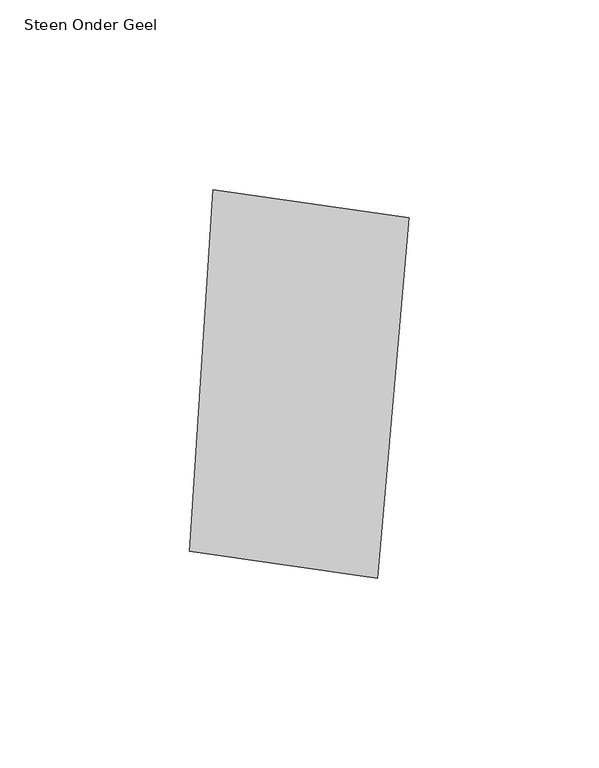
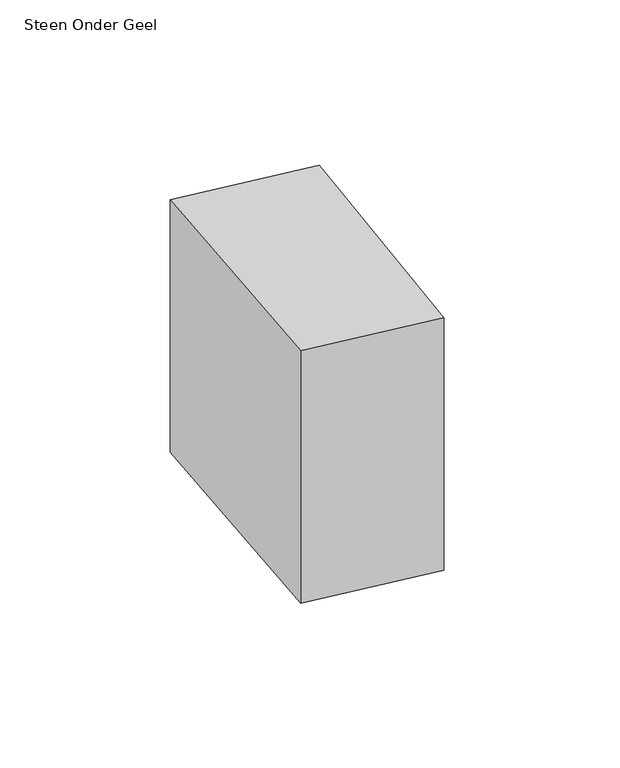
"""IFC4 building model written with IfcOpenShell, lengths in millimetres: proxy geometry, 00_GMA_steen_versie_4 : Steen Onder Geel."""

from ifc_helpers import new_model, si_unit, origin, origin_with_axes, place, context, project, spatial, polyline, outline, extrude, source, transform, mapped, element, save


def steen_onder_geel_60102d9a(model_context):
    return source(origin(), model_context, "Body", "SweptSolid", [
        extrude(outline(polyline([(104.4913091, 114.212909), (96.2842343, 19.4127052), (46.7864635, 26.4817004), (52.9037693, 121.5865884), (104.4913091, 114.212909)])), origin_with_axes(), (0.0, 0.0, 1.0), 100.0),
    ])


if __name__ == "__main__":
    model = new_model("IFC4")
    model_context = context("Model", 3, world=origin())
    ifc_project = project(units=[si_unit("LENGTHUNIT", "METRE", prefix="MILLI")], contexts=[model_context])
    site = spatial("IfcSite", under=ifc_project)
    building = spatial("IfcBuilding", under=site)
    placement = place(None, origin())
    steen_onder_geel_shape = steen_onder_geel_60102d9a(model_context)
    element("IfcBuildingElementProxy", 1, Name="00_GMA_steen_versie_4 : Steen Onder Geel", ObjectType="00_GMA_steen_versie_4 : Steen Onder Geel", at=placement, inside=building, context=model_context, shape_type="MappedRepresentation", body=[
        mapped(steen_onder_geel_shape, transform((0.0, 0.0, 0.0), x_axis=(1.0, 0.0, 0.0), y_axis=(0.0, 1.0, 0.0), z_axis=(0.0, 0.0, 1.0))),
    ])
    save(model, "model.ifc")

# Revit data of these elements
# Type "00_GMA_steen_versie_4 : Steen Onder Geel"
#   StootVoegHalfBoven [instance default] = 5 mm
#   StootVoegHalf [instance default] = 5 mm
#   StootVoegBreedteOnder = 10 mm
#   StootVoegBreedteBoven = 10 mm
#   Steendikte = 100 mm
#   LintVoegOnderHalf = 0 mm
#   LintVoegOnder = 0 mm
#   LintVoegBovenHalf = 5 mm
#   LintVoegBoven = 10 mm
#   materiaal = 21_steen_geel
#   MateriaalVoeg = none
#   Default Elevation = 0
# Element 1 (IfcBuildingElementProxy, "00_GMA_steen_versie_4 : Steen Onder Geel")
#   Materials on its faces: "21_steen_geel"
# Materials
#   "21_steen_geel": class "Unassigned", colour RGB 202 202 0, transparency 0, Cost = 0
